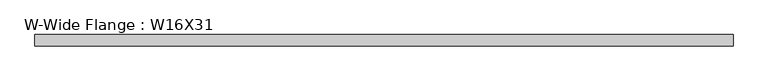
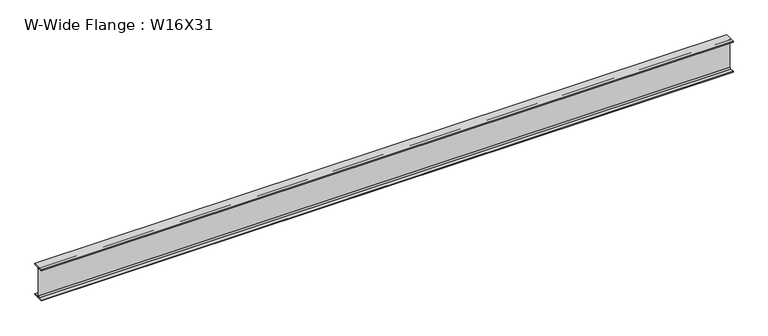
"""IFC4 building model written with IfcOpenShell, lengths in millimetres: beam geometry, W-Wide Flange : W16X31."""

from ifc_helpers import new_model, si_unit, point, frame, frame_2d, origin, place, context, project, spatial, polyline, circle_curve, trimmed, segment, composite_curve, outline, extrude, source, transform, mapped, element, save


def w_wide_flange_w16x31_1a0e2201(model_context):
    return source(origin(), model_context, "Body", "SweptSolid", [
        extrude(outline(composite_curve([segment(polyline([(70.231, -190.754), (70.231, -201.93), (-70.231, -201.93), (-70.231, -190.754), (-20.8915, -190.754)]), True, "CONTINUOUS"), segment(trimmed(circle_curve(frame_2d((-20.8915, -173.355)), 17.399), [point((-20.8915, -190.754))], [point((-3.4925, -173.355))], True, "CARTESIAN"), True, "CONTINUOUS"), segment(polyline([(-3.4925, -173.355), (-3.4925, 173.355)]), True, "CONTINUOUS"), segment(trimmed(circle_curve(frame_2d((-20.8915, 173.355)), 17.399), [point((-3.4925, 173.355))], [point((-20.8915, 190.754))], True, "CARTESIAN"), True, "CONTINUOUS"), segment(polyline([(-20.8915, 190.754), (-70.231, 190.754), (-70.231, 201.93), (70.231, 201.93), (70.231, 190.754), (20.8915, 190.754)]), True, "CONTINUOUS"), segment(trimmed(circle_curve(frame_2d((20.8915, 173.355)), 17.399), [point((20.8915, 190.754))], [point((3.4925, 173.355))], True, "CARTESIAN"), True, "CONTINUOUS"), segment(polyline([(3.4925, 173.355), (3.4925, -173.355)]), True, "CONTINUOUS"), segment(trimmed(circle_curve(frame_2d((20.8915, -173.355)), 17.399), [point((3.4925, -173.355))], [point((20.8915, -190.754))], True, "CARTESIAN"), True, "CONTINUOUS"), segment(polyline([(20.8915, -190.754), (70.231, -190.754)]), True, "CONTINUOUS")], self_intersect=False)), frame((-4213.6230758, 0.0, 0.0), z_axis=(1.0, 0.0, 0.0), x_axis=(0.0, 1.0, 0.0)), (0.0, 0.0, 1.0), 8543.7051516),
    ])


if __name__ == "__main__":
    model = new_model("IFC4")
    model_context = context("Model", 3, world=origin())
    ifc_project = project(units=[si_unit("LENGTHUNIT", "METRE", prefix="MILLI")], contexts=[model_context])
    site = spatial("IfcSite", under=ifc_project)
    building = spatial("IfcBuilding", under=site)
    placement = place(None, origin())
    w_wide_flange_w16x31_shape = w_wide_flange_w16x31_1a0e2201(model_context)
    element("IfcBeam", 1, ObjectType="W-Wide Flange : W16X31", at=placement, inside=building, context=model_context, shape_type="MappedRepresentation", body=[
        mapped(w_wide_flange_w16x31_shape, transform((0.0, 0.0, 0.0), x_axis=(1.0, 0.0, 0.0), y_axis=(0.0, 1.0, 0.0), z_axis=(0.0, 0.0, 1.0))),
    ])
    save(model, "model.ifc")

# Revit data of these elements
# Type "W-Wide Flange : W16X31"
#   Assembly Code = "B10"
#   W = 31
#   Start Extension Calculation [instance default] = 10' - 0"
#   Start Extension [instance default] = -0' - 0 1/2"
#   End Extension Calculation [instance default] = 10' - 0"
#   End Extension [instance default] = -0' - 0 1/2"
#   Length [instance default] = 5' - 0"
#   bf = 0' - 5.53"
#   d = 1' - 3.9"
#   k = 0' - 1 1/8"
#   k2 = 0' - 0.685"
#   tf = 0' - 0.44"
#   tw = 0' - 0.275"
#   A = 0.0634028 SF
#   Beam Material [instance default] = Metal - Steel - ASTM A992
# Element 1 (IfcBeam, "W-Wide Flange : W16X31")
#   Materials on its faces: "Metal - Steel - ASTM A992"
# Materials
#   "Metal - Steel - ASTM A992": class "Metal", colour RGB 128 0 0, transparency 0
